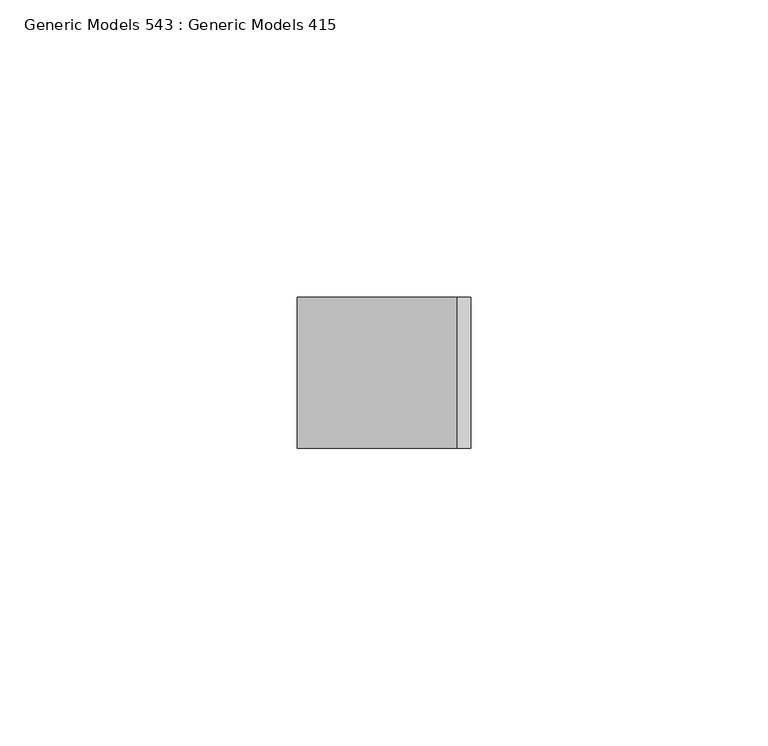
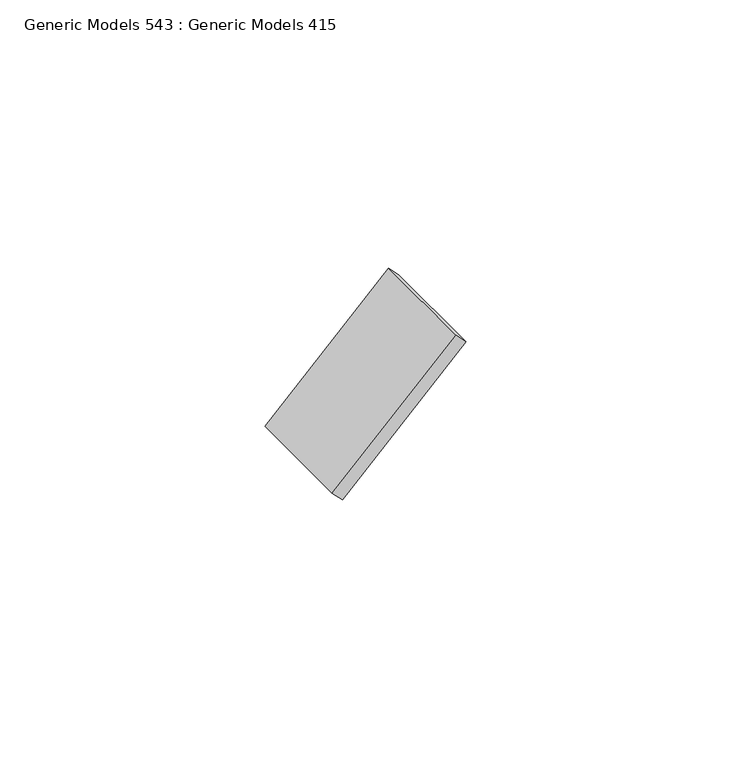
"""IFC4 building model written with IfcOpenShell, lengths in millimetres: proxy geometry, Generic Models 543 : Generic Models 415."""

from ifc_helpers import new_model, si_unit, frame, origin, place, context, project, spatial, polyline, outline, extrude, source, transform, mapped, element, save


def generic_models_543_generic_models_415_c80db9c1(model_context):
    return source(origin(), model_context, "Body", "SweptSolid", [
        extrude(outline(polyline([(0.0, -3.175), (0.0, 0.0), (25.4, 0.0), (25.4, -3.175), (0.0, -3.175)])), frame((7848.0411784, 4501.3863946, 124940.3849742), z_axis=(0.7071067811867181, 0.0, 0.707106781186377), x_axis=(0.0, -1.0, 0.0)), (0.0, 0.0, 1.0), 38.1),
    ])


if __name__ == "__main__":
    model = new_model("IFC4")
    model_context = context("Model", 3, world=origin())
    ifc_project = project(units=[si_unit("LENGTHUNIT", "METRE", prefix="MILLI")], contexts=[model_context])
    site = spatial("IfcSite", under=ifc_project)
    building = spatial("IfcBuilding", under=site)
    placement = place(None, origin())
    generic_models_543_generic_models_415_shape = generic_models_543_generic_models_415_c80db9c1(model_context)
    element("IfcBuildingElementProxy", 1, Name="Generic Models 543 : Generic Models 415", ObjectType="Generic Models 543 : Generic Models 415", at=placement, inside=building, context=model_context, shape_type="MappedRepresentation", body=[
        mapped(generic_models_543_generic_models_415_shape, transform((0.0, 0.0, 0.0), x_axis=(1.0, 0.0, 0.0), y_axis=(0.0, 1.0, 0.0), z_axis=(0.0, 0.0, 1.0))),
    ])
    save(model, "model.ifc")

# Revit data of these elements
# Element 1 (IfcBuildingElementProxy, "Generic Models 543 : Generic Models 415")
#   Materials on its faces: "_WELDED STEEL TABS FOR LOUVER ATTACHMENT"
# Materials
#   "_WELDED STEEL TABS FOR LOUVER ATTACHMENT": class "Metal", colour RGB 199 199 199, transparency 0, Description = "Structural steel 50ksi", Cost = 0
